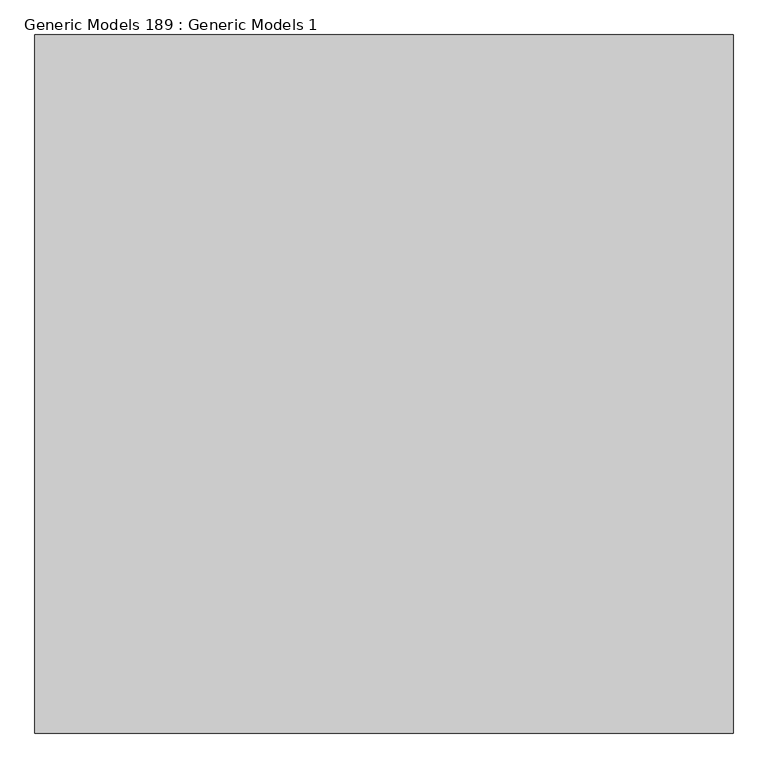
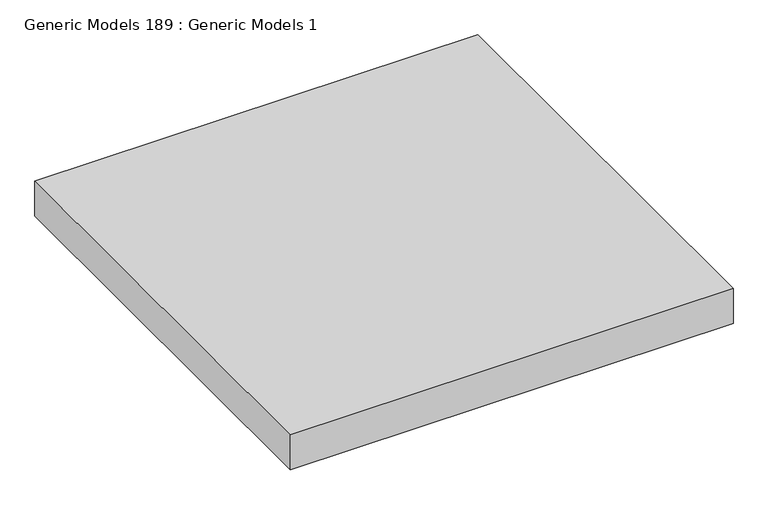
"""IFC4 building model written with IfcOpenShell, lengths in millimetres: proxy geometry, Generic Models 189 : Generic Models 1."""

from ifc_helpers import new_model, si_unit, frame, origin, place, context, project, spatial, polyline, outline, extrude, source, transform, mapped, element, save


def generic_models_189_generic_models_1_450c8840(model_context):
    return source(origin(), model_context, "Body", "SweptSolid", [
        extrude(outline(polyline([(50347.5625, 0.0), (49128.3625, 0.0), (49128.3625, 1219.2), (50347.5625, 1219.2), (50347.5625, 0.0)])), frame((0.0, 0.0, 2457.45), z_axis=(0.0, 0.0, 1.0), x_axis=(1.0, 0.0, 0.0)), (0.0, 0.0, 1.0), 101.6),
    ])


if __name__ == "__main__":
    model = new_model("IFC4")
    model_context = context("Model", 3, world=origin())
    ifc_project = project(units=[si_unit("LENGTHUNIT", "METRE", prefix="MILLI")], contexts=[model_context])
    site = spatial("IfcSite", under=ifc_project)
    building = spatial("IfcBuilding", under=site)
    placement = place(None, origin())
    generic_models_189_generic_models_1_shape = generic_models_189_generic_models_1_450c8840(model_context)
    element("IfcBuildingElementProxy", 1, Name="Generic Models 189 : Generic Models 1", ObjectType="Generic Models 189 : Generic Models 1", at=placement, inside=building, context=model_context, shape_type="MappedRepresentation", body=[
        mapped(generic_models_189_generic_models_1_shape, transform((0.0, 0.0, 0.0), x_axis=(1.0, 0.0, 0.0), y_axis=(0.0, 1.0, 0.0), z_axis=(0.0, 0.0, 1.0))),
    ])
    save(model, "model.ifc")

# Revit data of these elements
# Element 1 (IfcBuildingElementProxy, "Generic Models 189 : Generic Models 1")
#   Materials on its faces: "UNDERSIDE OF STRUCTURE"
# Materials
#   "UNDERSIDE OF STRUCTURE": class "Concrete", colour RGB 36 37 33, transparency 0, Description = "Lightweight concrete", Cost = 0
